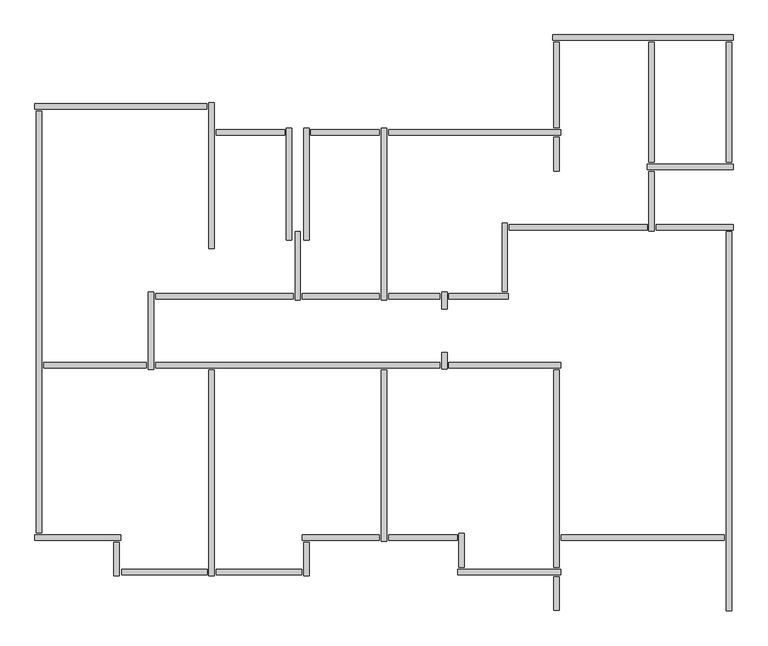
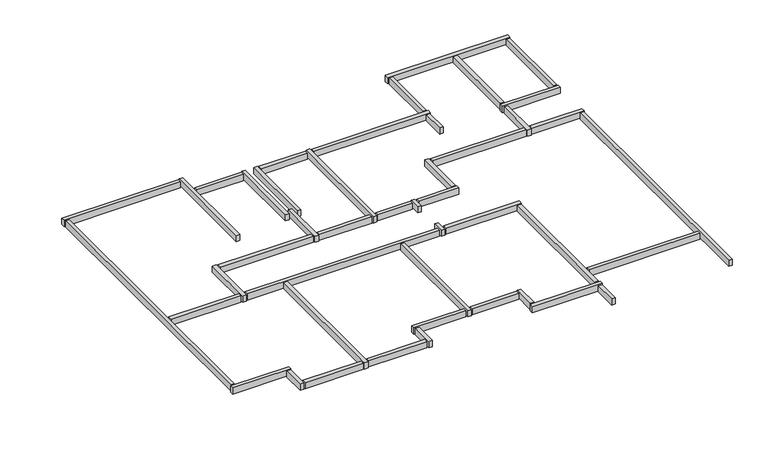
"""IFC4 building model written with IfcOpenShell, lengths in millimetres: beam geometry, Graute viga de respaldo22 : Graute viga de respaldo."""

import ifcopenshell
import ifcopenshell.guid

model = None  # the IFC model being written
_history = None  # IfcOwnerHistory: only IFC2X3 demands one
_inside = {}  # id of a spatial element -> (the spatial element, [elements in it])
_under = {}  # id of a project, library or spatial element -> (it, [spatial elements below it])
_declared = {}  # id of a project -> (the project, [libraries it declares])
_typed = {}  # id of a type object -> (the type object, [elements of that type])
_made_of = {}  # id of a material, layer set ... -> (it, [elements and type objects made of it])


def new_model(schema):
    """Start an empty IFC model of exactly this schema.

    Asked for "IFC4X3", IfcOpenShell would pick the latest addendum, in which some entities
    have other attributes; the version numbers below select the first issue.
    IFC2X3 requires an IfcOwnerHistory on every rooted entity: one is made here for all.
    """
    global model, _history
    if schema == "IFC4X3":
        model = ifcopenshell.file(schema_version=(4, 3, 0, 0))
    else:
        model = ifcopenshell.file(schema=schema)
    _inside.clear()
    _under.clear()
    _declared.clear()
    _typed.clear()
    _made_of.clear()
    _history = None
    if model.schema == "IFC2X3":
        org = make("IfcOrganization", Name="unknown")
        user = make(
            "IfcPersonAndOrganization",
            ThePerson=make("IfcPerson", FamilyName="unknown"),
            TheOrganization=org,
        )
        app = make(
            "IfcApplication",
            ApplicationDeveloper=org,
            Version="unknown",
            ApplicationFullName="unknown",
            ApplicationIdentifier="unknown",
        )
        _history = make(
            "IfcOwnerHistory",
            OwningUser=user,
            OwningApplication=app,
            ChangeAction="ADDED",
            CreationDate=0,
        )
    return model


def make(cls, **values):
    """One entity of the class cls with the attributes given. An attribute that is None is left unset."""
    return model.create_entity(
        cls, **{name: value for name, value in values.items() if value is not None}
    )


def rooted(cls, **values):
    """An entity with a GlobalId (a new one), such as an element, a storey or a relation."""
    return make(cls, GlobalId=ifcopenshell.guid.new(), OwnerHistory=_history, **values)


def si_unit(unit_type, name, prefix=None):
    """IfcSIUnit, for example si_unit("LENGTHUNIT", "METRE", prefix="MILLI")."""
    return make("IfcSIUnit", UnitType=unit_type, Prefix=prefix, Name=name)


def assignment(units):
    """IfcUnitAssignment: the units of a project."""
    return None if units is None else make("IfcUnitAssignment", Units=units)


def point(xyz):
    """IfcCartesianPoint."""
    return None if xyz is None else make("IfcCartesianPoint", Coordinates=xyz)


def direction(xyz):
    """IfcDirection."""
    return None if xyz is None else make("IfcDirection", DirectionRatios=xyz)


def frame(location, z_axis=None, x_axis=None):
    """IfcAxis2Placement3D, a coordinate frame: its origin and axes. An axis left out is left unset."""
    return make(
        "IfcAxis2Placement3D",
        Location=point(location),
        Axis=direction(z_axis),
        RefDirection=direction(x_axis),
    )


def origin():
    """The frame at (0, 0, 0) with its axes left unset."""
    return frame((0.0, 0.0, 0.0))


def place(relative_to, where):
    """IfcLocalPlacement: puts the frame where relative to a parent placement (None: the world)."""
    return make(
        "IfcLocalPlacement", PlacementRelTo=relative_to, RelativePlacement=where
    )


def context(
    kind, dimensions, precision=None, world=None, true_north=None, identifier=None
):
    """IfcGeometricRepresentationContext, for example the 3D "Model" context."""
    return make(
        "IfcGeometricRepresentationContext",
        ContextIdentifier=identifier,
        ContextType=kind,
        CoordinateSpaceDimension=dimensions,
        Precision=precision,
        WorldCoordinateSystem=world,
        TrueNorth=true_north,
    )


def project(units=None, contexts=None):
    """IfcProject with its units and contexts."""
    return rooted(
        "IfcProject",
        Name="project",
        RepresentationContexts=contexts,
        UnitsInContext=assignment(units),
    )


def spatial(cls, under=None, at=None, **own):
    """A site, building, storey or space (cls), placed at a placement, below another one or the project."""
    s = rooted(cls, ObjectPlacement=at, **own)
    if under is not None:
        _under.setdefault(under.id(), (under, []))[1].append(s)
    return s


def polyline(points):
    """IfcPolyline through the points."""
    return make("IfcPolyline", Points=[point(p) for p in points])


def outline(outer, holes=None, kind="AREA"):
    """IfcArbitraryClosedProfileDef: a profile drawn as a closed curve; with holes, ...WithVoids."""
    if holes is None:
        return make("IfcArbitraryClosedProfileDef", ProfileType=kind, OuterCurve=outer)
    return make(
        "IfcArbitraryProfileDefWithVoids",
        ProfileType=kind,
        OuterCurve=outer,
        InnerCurves=holes,
    )


def extrude(swept, where, along, depth):
    """IfcExtrudedAreaSolid: the profile swept, set in the frame where, extruded along a direction by depth."""
    return make(
        "IfcExtrudedAreaSolid",
        SweptArea=swept,
        Position=where,
        ExtrudedDirection=direction(along),
        Depth=depth,
    )


def shape(context_of_items, identifier, shape_type, items):
    """IfcShapeRepresentation: the items that make up one representation, for example the "Body"."""
    return make(
        "IfcShapeRepresentation",
        ContextOfItems=context_of_items,
        RepresentationIdentifier=identifier,
        RepresentationType=shape_type,
        Items=items,
    )


def source(mapping_origin, context_of_items, identifier, shape_type, items):
    """IfcRepresentationMap: a shape defined once, which mapped items show again and again."""
    return make(
        "IfcRepresentationMap",
        MappingOrigin=mapping_origin,
        MappedRepresentation=shape(context_of_items, identifier, shape_type, items),
    )


def transform(
    local_origin,
    x_axis=None,
    y_axis=None,
    z_axis=None,
    scale=None,
    scale2=None,
    scale3=None,
    uniform=True,
):
    """IfcCartesianTransformationOperator3D, or its non-uniform kind. x_axis, y_axis, z_axis: its Axis1, 2, 3."""
    if uniform:
        return make(
            "IfcCartesianTransformationOperator3D",
            Axis1=direction(x_axis),
            Axis2=direction(y_axis),
            LocalOrigin=point(local_origin),
            Scale=scale,
            Axis3=direction(z_axis),
        )
    return make(
        "IfcCartesianTransformationOperator3DnonUniform",
        Axis1=direction(x_axis),
        Axis2=direction(y_axis),
        LocalOrigin=point(local_origin),
        Scale=scale,
        Axis3=direction(z_axis),
        Scale2=scale2,
        Scale3=scale3,
    )


def mapped(mapping_source, mapping_target):
    """IfcMappedItem: shows the shape of a source again, moved by a transform."""
    return make(
        "IfcMappedItem", MappingSource=mapping_source, MappingTarget=mapping_target
    )


def made_of(thing, what):
    """Note that an element or type object is made of a material, layer set ...; save() writes the relation."""
    if what is not None:
        _made_of.setdefault(what.id(), (what, []))[1].append(thing)
    return thing


def element(
    cls,
    number,
    at=None,
    inside=None,
    cuts=None,
    type_object=None,
    material=None,
    context=None,
    identifier="Body",
    shape_type=None,
    held_by="IfcProductDefinitionShape",
    body=None,
    shapes=None,
    **own,
):
    """One element of the class cls, such as IfcWall. Its Tag is "e" and its number.

    at: its placement. inside: the storey or other place that contains it. cuts: it is an
    opening in that element (IfcRelVoidsElement). A single representation is given by context,
    identifier, shape_type and body (its items); several are given by shapes. held_by: the class
    of the entity that holds the representations. save() writes the other relations.
    """
    e = rooted(cls, Tag="e%d" % number, ObjectPlacement=at, **own)
    if body is not None:
        shapes = [shape(context, identifier, shape_type, body)]
    if shapes is not None:
        e.Representation = make(held_by, Representations=shapes)
    if inside is not None:
        _inside.setdefault(inside.id(), (inside, []))[1].append(e)
    if cuts is not None:
        rooted(
            "IfcRelVoidsElement", RelatingBuildingElement=cuts, RelatedOpeningElement=e
        )
    if type_object is not None:
        _typed.setdefault(type_object.id(), (type_object, []))[1].append(e)
    return made_of(e, material)


def aggregate(whole, parts):
    """IfcRelAggregates: a whole, such as a stair, and the parts it consists of."""
    return rooted("IfcRelAggregates", RelatingObject=whole, RelatedObjects=parts)


def save(model, path):
    """Write the relations noted so far, then the file.

    IfcRelAggregates (storeys below a building ...), IfcRelContainedInSpatialStructure (elements
    in a storey), IfcRelDefinesByType, IfcRelAssociatesMaterial and IfcRelDeclares: one each for
    every whole, place, type object, material and project.
    """
    for whole, parts in _under.values():
        aggregate(whole, parts)
    for where, things in _inside.values():
        rooted(
            "IfcRelContainedInSpatialStructure",
            RelatedElements=things,
            RelatingStructure=where,
        )
    for kind, things in _typed.values():
        rooted("IfcRelDefinesByType", RelatedObjects=things, RelatingType=kind)
    for what, things in _made_of.values():
        rooted("IfcRelAssociatesMaterial", RelatedObjects=things, RelatingMaterial=what)
    for by, libraries in _declared.values():
        rooted("IfcRelDeclares", RelatingContext=by, RelatedDefinitions=libraries)
    model.write(path)


def beam_285e0457(model_context):
    return source(origin(), model_context, "Body", "SweptSolid", [
        extrude(outline(polyline([(-75401.7587292, 57502.4278788), (-75401.7587292, 57408.4278788), (-76591.7587292, 57408.4278788), (-76591.7587292, 57502.4278788), (-75401.7587292, 57502.4278788)])), frame((0.0, 0.0, 17632.9999999), z_axis=(0.0, 0.0, 1.0), x_axis=(1.0, 0.0, 0.0)), (0.0, 0.0, 1.0), 167.0),
        extrude(outline(polyline([(-73751.7587292, 57502.4278788), (-73751.7587292, 57408.4278788), (-74941.7587292, 57408.4278788), (-74941.7587292, 57502.4278788), (-73751.7587292, 57502.4278788)])), frame((0.0, 0.0, 17632.9999999), z_axis=(0.0, 0.0, 1.0), x_axis=(1.0, 0.0, 0.0)), (0.0, 0.0, 1.0), 167.0),
        extrude(outline(polyline([(-77801.7587292, 53452.4278788), (-77801.7587292, 53358.4278788), (-79591.7587292, 53358.4278788), (-79591.7587292, 53452.4278788), (-77801.7587292, 53452.4278788)])), frame((0.0, 0.0, 17632.9999999), z_axis=(0.0, 0.0, 1.0), x_axis=(1.0, 0.0, 0.0)), (0.0, 0.0, 1.0), 167.0),
        extrude(outline(polyline([(-72401.7587292, 50452.4278788), (-72401.7587292, 50358.4278788), (-73591.7587292, 50358.4278788), (-73591.7587292, 50452.4278788), (-72401.7587292, 50452.4278788)])), frame((0.0, 0.0, 17632.9999999), z_axis=(0.0, 0.0, 1.0), x_axis=(1.0, 0.0, 0.0)), (0.0, 0.0, 1.0), 167.0),
        extrude(outline(polyline([(-72368.7587292, 50475.4278788), (-72274.7587292, 50475.4278788), (-72274.7587292, 49885.4278788), (-72368.7587292, 49885.4278788), (-72368.7587292, 50475.4278788)])), frame((0.0, 0.0, 17632.9999999), z_axis=(0.0, 0.0, 1.0), x_axis=(1.0, 0.0, 0.0)), (0.0, 0.0, 1.0), 167.0),
        extrude(outline(polyline([(-70601.7587292, 49852.4278788), (-70601.7587292, 49758.4278788), (-72391.7587292, 49758.4278788), (-72391.7587292, 49852.4278788), (-70601.7587292, 49852.4278788)])), frame((0.0, 0.0, 17632.9999999), z_axis=(0.0, 0.0, 1.0), x_axis=(1.0, 0.0, 0.0)), (0.0, 0.0, 1.0), 167.0),
        extrude(outline(polyline([(-72574.7587292, 53335.4278788), (-72668.7587292, 53335.4278788), (-72668.7587292, 53625.4278788), (-72574.7587292, 53625.4278788), (-72574.7587292, 53335.4278788)])), frame((0.0, 0.0, 17632.9999999), z_axis=(0.0, 0.0, 1.0), x_axis=(1.0, 0.0, 0.0)), (0.0, 0.0, 1.0), 167.0),
        extrude(outline(polyline([(-75251.7587292, 54652.4278788), (-75251.7587292, 54558.4278788), (-77641.7587292, 54558.4278788), (-77641.7587292, 54652.4278788), (-75251.7587292, 54652.4278788)])), frame((0.0, 0.0, 17632.9999999), z_axis=(0.0, 0.0, 1.0), x_axis=(1.0, 0.0, 0.0)), (0.0, 0.0, 1.0), 167.0),
        extrude(outline(polyline([(-73751.7587292, 54652.4278788), (-73751.7587292, 54558.4278788), (-75091.7587292, 54558.4278788), (-75091.7587292, 54652.4278788), (-73751.7587292, 54652.4278788)])), frame((0.0, 0.0, 17632.9999999), z_axis=(0.0, 0.0, 1.0), x_axis=(1.0, 0.0, 0.0)), (0.0, 0.0, 1.0), 167.0),
        extrude(outline(polyline([(-72701.7587292, 54652.4278788), (-72701.7587292, 54558.4278788), (-73591.7587292, 54558.4278788), (-73591.7587292, 54652.4278788), (-72701.7587292, 54652.4278788)])), frame((0.0, 0.0, 17632.9999999), z_axis=(0.0, 0.0, 1.0), x_axis=(1.0, 0.0, 0.0)), (0.0, 0.0, 1.0), 167.0),
        extrude(outline(polyline([(-72574.7587292, 54385.4278788), (-72668.7587292, 54385.4278788), (-72668.7587292, 54675.4278788), (-72574.7587292, 54675.4278788), (-72574.7587292, 54385.4278788)])), frame((0.0, 0.0, 17632.9999999), z_axis=(0.0, 0.0, 1.0), x_axis=(1.0, 0.0, 0.0)), (0.0, 0.0, 1.0), 167.0),
        extrude(outline(polyline([(-71511.7587292, 54652.4278788), (-71511.7587292, 54558.4278788), (-72541.7587292, 54558.4278788), (-72541.7587292, 54652.4278788), (-71511.7587292, 54652.4278788)])), frame((0.0, 0.0, 17632.9999999), z_axis=(0.0, 0.0, 1.0), x_axis=(1.0, 0.0, 0.0)), (0.0, 0.0, 1.0), 167.0),
        extrude(outline(polyline([(-71618.7587292, 55875.4278788), (-71524.7587292, 55875.4278788), (-71524.7587292, 54685.4278788), (-71618.7587292, 54685.4278788), (-71618.7587292, 55875.4278788)])), frame((0.0, 0.0, 17632.9999999), z_axis=(0.0, 0.0, 1.0), x_axis=(1.0, 0.0, 0.0)), (0.0, 0.0, 1.0), 167.0),
        extrude(outline(polyline([(-69091.7587292, 55852.4278788), (-69091.7587292, 55758.4278788), (-71491.7587292, 55758.4278788), (-71491.7587292, 55852.4278788), (-69091.7587292, 55852.4278788)])), frame((0.0, 0.0, 17632.9999999), z_axis=(0.0, 0.0, 1.0), x_axis=(1.0, 0.0, 0.0)), (0.0, 0.0, 1.0), 167.0),
        extrude(outline(polyline([(-73624.7587292, 54540.4278788), (-73718.7587292, 54540.4278788), (-73718.7587292, 57525.4278788), (-73624.7587292, 57525.4278788), (-73624.7587292, 54540.4278788)])), frame((0.0, 0.0, 17632.9999999), z_axis=(0.0, 0.0, 1.0), x_axis=(1.0, 0.0, 0.0)), (0.0, 0.0, 1.0), 167.0),
        extrude(outline(polyline([(-70601.7587292, 57502.4278788), (-70601.7587292, 57408.4278788), (-73591.7587292, 57408.4278788), (-73591.7587292, 57502.4278788), (-70601.7587292, 57502.4278788)])), frame((0.0, 0.0, 17632.9999999), z_axis=(0.0, 0.0, 1.0), x_axis=(1.0, 0.0, 0.0)), (0.0, 0.0, 1.0), 167.0),
        extrude(outline(polyline([(-70624.7587292, 56785.4278788), (-70718.7587292, 56785.4278788), (-70718.7587292, 57375.4278788), (-70624.7587292, 57375.4278788), (-70624.7587292, 56785.4278788)])), frame((0.0, 0.0, 17632.9999999), z_axis=(0.0, 0.0, 1.0), x_axis=(1.0, 0.0, 0.0)), (0.0, 0.0, 1.0), 167.0),
        extrude(outline(polyline([(-70718.7587292, 59025.4278788), (-70624.7587292, 59025.4278788), (-70624.7587292, 57535.4278788), (-70718.7587292, 57535.4278788), (-70718.7587292, 59025.4278788)])), frame((0.0, 0.0, 17632.9999999), z_axis=(0.0, 0.0, 1.0), x_axis=(1.0, 0.0, 0.0)), (0.0, 0.0, 1.0), 167.0),
        extrude(outline(polyline([(-67718.7587292, 59025.4278788), (-67624.7587292, 59025.4278788), (-67624.7587292, 56935.4278788), (-67718.7587292, 56935.4278788), (-67718.7587292, 59025.4278788)])), frame((0.0, 0.0, 17632.9999999), z_axis=(0.0, 0.0, 1.0), x_axis=(1.0, 0.0, 0.0)), (0.0, 0.0, 1.0), 167.0),
        extrude(outline(polyline([(-69068.7587292, 59025.4278788), (-68974.7587292, 59025.4278788), (-68974.7587292, 56935.4278788), (-69068.7587292, 56935.4278788), (-69068.7587292, 59025.4278788)])), frame((0.0, 0.0, 17632.9999999), z_axis=(0.0, 0.0, 1.0), x_axis=(1.0, 0.0, 0.0)), (0.0, 0.0, 1.0), 167.0),
        extrude(outline(polyline([(-68974.7587292, 55735.4278788), (-69068.7587292, 55735.4278788), (-69068.7587292, 56775.4278788), (-68974.7587292, 56775.4278788), (-68974.7587292, 55735.4278788)])), frame((0.0, 0.0, 17632.9999999), z_axis=(0.0, 0.0, 1.0), x_axis=(1.0, 0.0, 0.0)), (0.0, 0.0, 1.0), 167.0),
        extrude(outline(polyline([(-67751.7587292, 50452.4278788), (-67751.7587292, 50358.4278788), (-70591.7587292, 50358.4278788), (-70591.7587292, 50452.4278788), (-67751.7587292, 50452.4278788)])), frame((0.0, 0.0, 17632.9999999), z_axis=(0.0, 0.0, 1.0), x_axis=(1.0, 0.0, 0.0)), (0.0, 0.0, 1.0), 167.0),
        extrude(outline(polyline([(-70718.7587292, 53325.4278788), (-70624.7587292, 53325.4278788), (-70624.7587292, 49885.4278788), (-70718.7587292, 49885.4278788), (-70718.7587292, 53325.4278788)])), frame((0.0, 0.0, 17632.9999999), z_axis=(0.0, 0.0, 1.0), x_axis=(1.0, 0.0, 0.0)), (0.0, 0.0, 1.0), 167.0),
        extrude(outline(polyline([(-70601.7587292, 53452.4278788), (-70601.7587292, 53358.4278788), (-72541.7587292, 53358.4278788), (-72541.7587292, 53452.4278788), (-70601.7587292, 53452.4278788)])), frame((0.0, 0.0, 17632.9999999), z_axis=(0.0, 0.0, 1.0), x_axis=(1.0, 0.0, 0.0)), (0.0, 0.0, 1.0), 167.0),
        extrude(outline(polyline([(-72701.7587292, 53452.4278788), (-72701.7587292, 53358.4278788), (-77641.7587292, 53358.4278788), (-77641.7587292, 53452.4278788), (-72701.7587292, 53452.4278788)])), frame((0.0, 0.0, 17632.9999999), z_axis=(0.0, 0.0, 1.0), x_axis=(1.0, 0.0, 0.0)), (0.0, 0.0, 1.0), 167.0),
        extrude(outline(polyline([(-73624.7587292, 50335.4278788), (-73718.7587292, 50335.4278788), (-73718.7587292, 53325.4278788), (-73624.7587292, 53325.4278788), (-73624.7587292, 50335.4278788)])), frame((0.0, 0.0, 17632.9999999), z_axis=(0.0, 0.0, 1.0), x_axis=(1.0, 0.0, 0.0)), (0.0, 0.0, 1.0), 167.0),
        extrude(outline(polyline([(-75091.7587292, 50358.4278788), (-75091.7587292, 50452.4278788), (-73751.7587292, 50452.4278788), (-73751.7587292, 50358.4278788), (-75091.7587292, 50358.4278788)])), frame((0.0, 0.0, 17632.9999999), z_axis=(0.0, 0.0, 1.0), x_axis=(1.0, 0.0, 0.0)), (0.0, 0.0, 1.0), 167.0),
        extrude(outline(polyline([(-74974.7587292, 49735.4278788), (-75068.7587292, 49735.4278788), (-75068.7587292, 50325.4278788), (-74974.7587292, 50325.4278788), (-74974.7587292, 49735.4278788)])), frame((0.0, 0.0, 17632.9999999), z_axis=(0.0, 0.0, 1.0), x_axis=(1.0, 0.0, 0.0)), (0.0, 0.0, 1.0), 167.0),
        extrude(outline(polyline([(-75101.7587292, 49852.4278788), (-75101.7587292, 49758.4278788), (-76591.7587292, 49758.4278788), (-76591.7587292, 49852.4278788), (-75101.7587292, 49852.4278788)])), frame((0.0, 0.0, 17632.9999999), z_axis=(0.0, 0.0, 1.0), x_axis=(1.0, 0.0, 0.0)), (0.0, 0.0, 1.0), 167.0),
        extrude(outline(polyline([(-78230.736554, 49758.4278788), (-78230.736554, 49853.4278788), (-76741.7587292, 49853.4278788), (-76741.7587292, 49758.4278788), (-78230.736554, 49758.4278788)])), frame((0.0, 0.0, 17617.1856208), z_axis=(0.0, 0.0, 1.0), x_axis=(1.0, 0.0, 0.0)), (0.0, 0.0, 1.0), 165.0),
        extrude(outline(polyline([(-79718.7587292, 57825.4278788), (-79624.7587292, 57825.4278788), (-79624.7587292, 50485.4278788), (-79718.7587292, 50485.4278788), (-79718.7587292, 57825.4278788)])), frame((0.0, 0.0, 17632.9999999), z_axis=(0.0, 0.0, 1.0), x_axis=(1.0, 0.0, 0.0)), (0.0, 0.0, 1.0), 167.0),
        extrude(outline(polyline([(-77768.7587292, 54675.4278788), (-77674.7587292, 54675.4278788), (-77674.7587292, 53330.0746661), (-77768.7587292, 53330.0746661), (-77768.7587292, 54675.4278788)])), frame((0.0, 0.0, 17632.9999999), z_axis=(0.0, 0.0, 1.0), x_axis=(1.0, 0.0, 0.0)), (0.0, 0.0, 1.0), 167.0),
        extrude(outline(polyline([(-75218.7587292, 55725.4278788), (-75124.7587292, 55725.4278788), (-75124.7587292, 54535.4278788), (-75218.7587292, 54535.4278788), (-75218.7587292, 55725.4278788)])), frame((0.0, 0.0, 17632.9999999), z_axis=(0.0, 0.0, 1.0), x_axis=(1.0, 0.0, 0.0)), (0.0, 0.0, 1.0), 167.0),
        extrude(outline(polyline([(-75368.7587292, 57525.4278788), (-75274.7587292, 57525.4278788), (-75274.7587292, 55585.4278788), (-75368.7587292, 55585.4278788), (-75368.7587292, 57525.4278788)])), frame((0.0, 0.0, 17632.9999999), z_axis=(0.0, 0.0, 1.0), x_axis=(1.0, 0.0, 0.0)), (0.0, 0.0, 1.0), 167.0),
        extrude(outline(polyline([(-75068.7587292, 57525.4278788), (-74974.7587292, 57525.4278788), (-74974.7587292, 55585.4278788), (-75068.7587292, 55585.4278788), (-75068.7587292, 57525.4278788)])), frame((0.0, 0.0, 17632.9999999), z_axis=(0.0, 0.0, 1.0), x_axis=(1.0, 0.0, 0.0)), (0.0, 0.0, 1.0), 167.0),
        extrude(outline(polyline([(-76718.7587292, 57975.4278788), (-76624.7587292, 57975.4278788), (-76624.7587292, 55435.4278788), (-76718.7587292, 55435.4278788), (-76718.7587292, 57975.4278788)])), frame((0.0, 0.0, 17632.9999999), z_axis=(0.0, 0.0, 1.0), x_axis=(1.0, 0.0, 0.0)), (0.0, 0.0, 1.0), 167.0),
        extrude(outline(polyline([(-79741.7587292, 57858.4278788), (-79741.7587292, 57952.4278788), (-76751.7587292, 57952.4278788), (-76751.7587292, 57858.4278788), (-79741.7587292, 57858.4278788)])), frame((0.0, 0.0, 17632.9999999), z_axis=(0.0, 0.0, 1.0), x_axis=(1.0, 0.0, 0.0)), (0.0, 0.0, 1.0), 167.0),
        extrude(outline(polyline([(-78274.7587292, 49735.4278788), (-78368.7587292, 49735.4278788), (-78368.7587292, 50325.4278788), (-78274.7587292, 50325.4278788), (-78274.7587292, 49735.4278788)])), frame((0.0, 0.0, 17632.9999999), z_axis=(0.0, 0.0, 1.0), x_axis=(1.0, 0.0, 0.0)), (0.0, 0.0, 1.0), 167.0),
        extrude(outline(polyline([(-78251.7587292, 50452.4278788), (-78251.7587292, 50358.4278788), (-79741.7587292, 50358.4278788), (-79741.7587292, 50452.4278788), (-78251.7587292, 50452.4278788)])), frame((0.0, 0.0, 17632.9999999), z_axis=(0.0, 0.0, 1.0), x_axis=(1.0, 0.0, 0.0)), (0.0, 0.0, 1.0), 167.0),
        extrude(outline(polyline([(-76624.7587292, 49735.4278788), (-76718.7587292, 49735.4278788), (-76718.7587292, 53325.4278788), (-76624.7587292, 53325.4278788), (-76624.7587292, 49735.4278788)])), frame((0.0, 0.0, 17632.9999999), z_axis=(0.0, 0.0, 1.0), x_axis=(1.0, 0.0, 0.0)), (0.0, 0.0, 1.0), 167.0),
        extrude(outline(polyline([(-70624.7587292, 49135.4278788), (-70718.7587292, 49135.4278788), (-70718.7587292, 49725.4278788), (-70624.7587292, 49725.4278788), (-70624.7587292, 49135.4278788)])), frame((0.0, 0.0, 17632.9999999), z_axis=(0.0, 0.0, 1.0), x_axis=(1.0, 0.0, 0.0)), (0.0, 0.0, 1.0), 167.0),
        extrude(outline(polyline([(-67601.7587292, 56902.4278788), (-67601.7587292, 56808.4278788), (-69091.7587292, 56808.4278788), (-69091.7587292, 56902.4278788), (-67601.7587292, 56902.4278788)])), frame((0.0, 0.0, 17632.9999999), z_axis=(0.0, 0.0, 1.0), x_axis=(1.0, 0.0, 0.0)), (0.0, 0.0, 1.0), 167.0),
        extrude(outline(polyline([(-67601.7587292, 59152.4278788), (-67601.7587292, 59058.4278788), (-70741.7587292, 59058.4278788), (-70741.7587292, 59152.4278788), (-67601.7587292, 59152.4278788)])), frame((0.0, 0.0, 17632.9999999), z_axis=(0.0, 0.0, 1.0), x_axis=(1.0, 0.0, 0.0)), (0.0, 0.0, 1.0), 167.0),
        extrude(outline(polyline([(-67601.7587292, 55852.4278788), (-67601.7587292, 55758.4278788), (-68941.7587292, 55758.4278788), (-68941.7587292, 55852.4278788), (-67601.7587292, 55852.4278788)])), frame((0.0, 0.0, 17632.9999999), z_axis=(0.0, 0.0, 1.0), x_axis=(1.0, 0.0, 0.0)), (0.0, 0.0, 1.0), 167.0),
        extrude(outline(polyline([(-67624.7587292, 49132.8979841), (-67718.7587292, 49132.8979841), (-67718.7587292, 55725.4278788), (-67624.7587292, 55725.4278788), (-67624.7587292, 49132.8979841)])), frame((0.0, 0.0, 17632.9999999), z_axis=(0.0, 0.0, 1.0), x_axis=(1.0, 0.0, 0.0)), (0.0, 0.0, 1.0), 167.0),
    ])


if __name__ == "__main__":
    model = new_model("IFC4")
    model_context = context("Model", 3, world=origin())
    ifc_project = project(units=[si_unit("LENGTHUNIT", "METRE", prefix="MILLI")], contexts=[model_context])
    site = spatial("IfcSite", under=ifc_project)
    building = spatial("IfcBuilding", under=site)
    placement = place(None, origin())
    beam_shape = beam_285e0457(model_context)
    element("IfcBeam", 1, ObjectType="Graute viga de respaldo22 : Graute viga de respaldo", at=placement, inside=building, context=model_context, shape_type="MappedRepresentation", body=[
        mapped(beam_shape, transform((0.0, 0.0, 0.0), x_axis=(1.0, 0.0, 0.0), y_axis=(0.0, 1.0, 0.0), z_axis=(0.0, 0.0, 1.0))),
    ])
    save(model, "model.ifc")

# Revit data of these elements
# Element 1 (IfcBeam, "Graute viga de respaldo22 : Graute viga de respaldo")
#   Materials on its faces: "Concreto, Faixa de areia/cimento"
# Materials
#   "Concreto, Faixa de areia/cimento": class "Concreto", colour RGB 127 127 127, transparency 0, Description = "Revestimento de laje de concreto", Cost = 0
